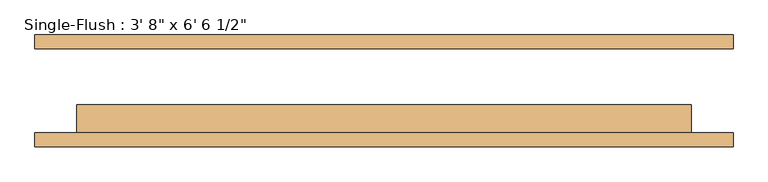
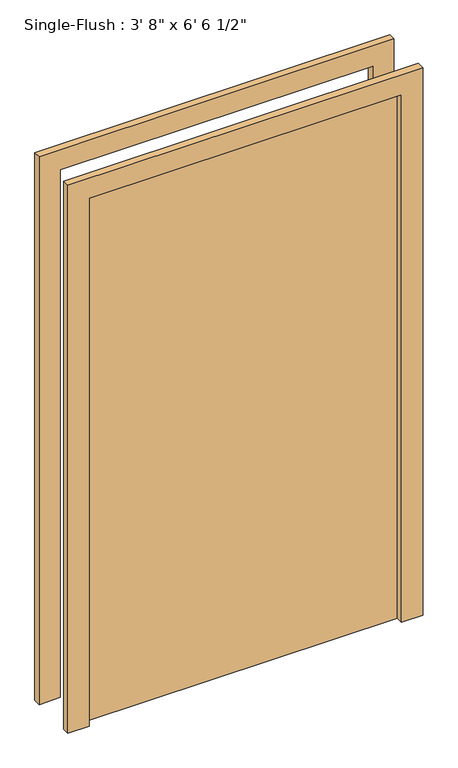
"""IFC4 building model written with IfcOpenShell, lengths in millimetres: door geometry."""

from ifc_helpers import new_model, si_unit, frame, origin, origin_with_axes, place, context, project, spatial, polyline, outline, extrude, source, transform, mapped, element, save


def door_05aa22aa(model_context):
    return source(origin(), model_context, "Body", "SweptSolid", [
        extrude(outline(polyline([(2070.1, -635.0), (0.0, -635.0), (0.0, -558.8), (1993.9, -558.8), (1993.9, 558.8), (0.0, 558.8), (0.0, 635.0), (2070.1, 635.0), (2070.1, -635.0)])), frame((0.0, -101.6, 0.0), z_axis=(0.0, 1.0, 0.0), x_axis=(0.0, 0.0, 1.0)), (0.0, 0.0, 1.0), 25.4),
        extrude(outline(polyline([(2070.1, 635.0), (2070.1, -635.0), (0.0, -635.0), (0.0, -558.8), (1993.9, -558.8), (1993.9, 558.8), (0.0, 558.8), (0.0, 635.0), (2070.1, 635.0)])), frame((0.0, 76.2, 0.0), z_axis=(0.0, 1.0, 0.0), x_axis=(0.0, 0.0, 1.0)), (0.0, 0.0, 1.0), 25.4),
        extrude(outline(polyline([(558.8, -25.4), (558.8, -76.2), (-558.8, -76.2), (-558.8, -25.4), (558.8, -25.4)])), origin_with_axes(), (0.0, 0.0, 1.0), 1993.9),
    ])


if __name__ == "__main__":
    model = new_model("IFC4")
    model_context = context("Model", 3, world=origin())
    ifc_project = project(units=[si_unit("LENGTHUNIT", "METRE", prefix="MILLI")], contexts=[model_context])
    site = spatial("IfcSite", under=ifc_project)
    building = spatial("IfcBuilding", under=site)
    placement = place(None, origin())
    door_shape = door_05aa22aa(model_context)
    element("IfcDoor", 1, ObjectType="Single-Flush : 3' 8\" x 6' 6 1/2\"", at=placement, inside=building, context=model_context, shape_type="MappedRepresentation", body=[
        mapped(door_shape, transform((0.0, 0.0, 0.0), x_axis=(1.0, 0.0, 0.0), y_axis=(0.0, 1.0, 0.0), z_axis=(0.0, 0.0, 1.0))),
    ])
    save(model, "model.ifc")

# Revit data of these elements
# Project information
#   Project Issue Date = "Issue Date"
#   Project Status = "Project Status"
#   Client Name = "Owner"
#   Project Address = "Enter address here"
#   Project Name = "Project Name"
#   Project Number = "Project Number"
# Type "Single-Flush : 3' 8\" x 6' 6 1/2\""
#   Type Mark = "10"
#   Assembly Code = "C1020"
#   Thickness = 0' - 2"
#   Height = 6' - 6 1/2"
#   Trim Projection Ext = 0' - 1"
#   Trim Projection Int = 0' - 1"
#   Trim Width = 0' - 3"
#   Width = 3' - 8"
#   Door Material = Door - Panel
#   Frame Material = Door - Frame
#   Function = (empty or 0)
#   Wall Closure = (empty or 0)
# Element 1 (IfcDoor, "Single-Flush : 3' 8\" x 6' 6 1/2\"")
#   Materials on its faces: "Door - Frame", "Door - Panel"
# Materials
#   "Door - Panel": class "Wood", colour RGB 114 82 51, transparency 0
#   "Door - Frame": class "Miscellaneous", colour RGB 153 76 43, transparency 0
